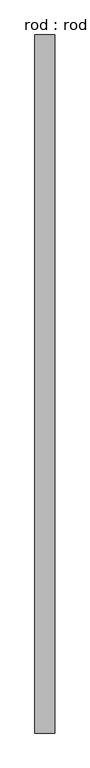
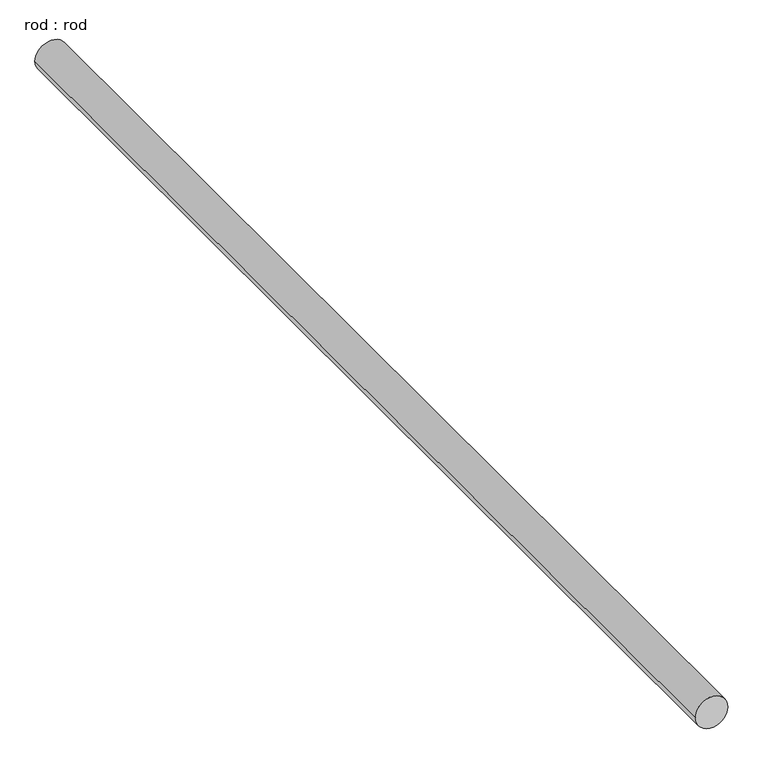
"""IFC4 building model written with IfcOpenShell, lengths in millimetres: proxy geometry, rod : rod."""

from ifc_helpers import new_model, si_unit, point, frame, frame_2d, origin, place, context, project, spatial, circle_curve, trimmed, segment, composite_curve, outline, extrude, source, transform, mapped, element, save


def rod_rod_749619da(model_context):
    return source(origin(), model_context, "Body", "SweptSolid", [
        extrude(outline(composite_curve([segment(trimmed(circle_curve(frame_2d((0.0108462, 0.0)), 200.0), [point((0.0108462, 200.0))], [point((0.0108462, -200.0))], False, "CARTESIAN"), True, "CONTINUOUS"), segment(trimmed(circle_curve(frame_2d((0.0108462, 0.0)), 200.0), [point((0.0108462, -200.0))], [point((0.0108462, 200.0))], False, "CARTESIAN"), True, "CONTINUOUS")], self_intersect=False)), frame((0.0, -2907.2713847, 0.0), z_axis=(0.0, 1.0, 0.0), x_axis=(0.0, 0.0, 1.0)), (0.0, 0.0, 1.0), 14000.0),
    ])


if __name__ == "__main__":
    model = new_model("IFC4")
    model_context = context("Model", 3, world=origin())
    ifc_project = project(units=[si_unit("LENGTHUNIT", "METRE", prefix="MILLI")], contexts=[model_context])
    site = spatial("IfcSite", under=ifc_project)
    building = spatial("IfcBuilding", under=site)
    placement = place(None, origin())
    rod_rod_shape = rod_rod_749619da(model_context)
    element("IfcBuildingElementProxy", 1, Name="rod : rod", ObjectType="rod : rod", at=placement, inside=building, context=model_context, shape_type="MappedRepresentation", body=[
        mapped(rod_rod_shape, transform((0.0, 0.0, 0.0), x_axis=(1.0, 0.0, 0.0), y_axis=(0.0, 1.0, 0.0), z_axis=(0.0, 0.0, 1.0))),
    ])
    save(model, "model.ifc")

# Revit data of these elements
# Type "rod : rod"
#   Default Elevation = 0
